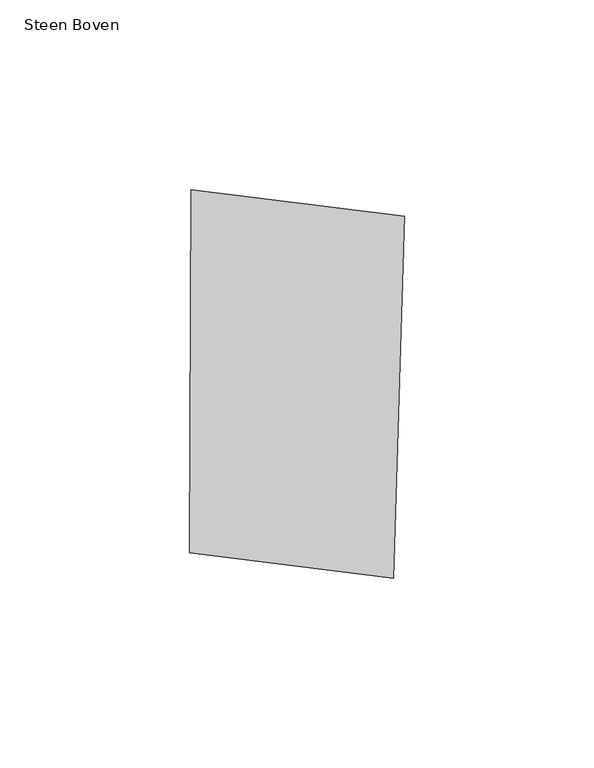
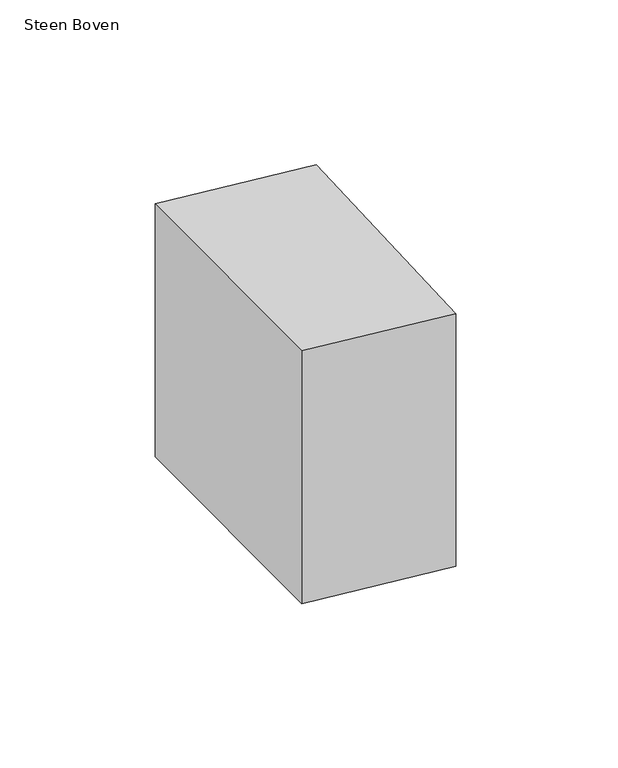
"""IFC4 building model written with IfcOpenShell, lengths in millimetres: proxy geometry, 00_GMA_steen_versie_4 : Steen Boven."""

import ifcopenshell
import ifcopenshell.guid

model = None  # the IFC model being written
_history = None  # IfcOwnerHistory: only IFC2X3 demands one
_inside = {}  # id of a spatial element -> (the spatial element, [elements in it])
_under = {}  # id of a project, library or spatial element -> (it, [spatial elements below it])
_declared = {}  # id of a project -> (the project, [libraries it declares])
_typed = {}  # id of a type object -> (the type object, [elements of that type])
_made_of = {}  # id of a material, layer set ... -> (it, [elements and type objects made of it])


def new_model(schema):
    """Start an empty IFC model of exactly this schema.

    Asked for "IFC4X3", IfcOpenShell would pick the latest addendum, in which some entities
    have other attributes; the version numbers below select the first issue.
    IFC2X3 requires an IfcOwnerHistory on every rooted entity: one is made here for all.
    """
    global model, _history
    if schema == "IFC4X3":
        model = ifcopenshell.file(schema_version=(4, 3, 0, 0))
    else:
        model = ifcopenshell.file(schema=schema)
    _inside.clear()
    _under.clear()
    _declared.clear()
    _typed.clear()
    _made_of.clear()
    _history = None
    if model.schema == "IFC2X3":
        org = make("IfcOrganization", Name="unknown")
        user = make(
            "IfcPersonAndOrganization",
            ThePerson=make("IfcPerson", FamilyName="unknown"),
            TheOrganization=org,
        )
        app = make(
            "IfcApplication",
            ApplicationDeveloper=org,
            Version="unknown",
            ApplicationFullName="unknown",
            ApplicationIdentifier="unknown",
        )
        _history = make(
            "IfcOwnerHistory",
            OwningUser=user,
            OwningApplication=app,
            ChangeAction="ADDED",
            CreationDate=0,
        )
    return model


def make(cls, **values):
    """One entity of the class cls with the attributes given. An attribute that is None is left unset."""
    return model.create_entity(
        cls, **{name: value for name, value in values.items() if value is not None}
    )


def rooted(cls, **values):
    """An entity with a GlobalId (a new one), such as an element, a storey or a relation."""
    return make(cls, GlobalId=ifcopenshell.guid.new(), OwnerHistory=_history, **values)


def si_unit(unit_type, name, prefix=None):
    """IfcSIUnit, for example si_unit("LENGTHUNIT", "METRE", prefix="MILLI")."""
    return make("IfcSIUnit", UnitType=unit_type, Prefix=prefix, Name=name)


def assignment(units):
    """IfcUnitAssignment: the units of a project."""
    return None if units is None else make("IfcUnitAssignment", Units=units)


def point(xyz):
    """IfcCartesianPoint."""
    return None if xyz is None else make("IfcCartesianPoint", Coordinates=xyz)


def direction(xyz):
    """IfcDirection."""
    return None if xyz is None else make("IfcDirection", DirectionRatios=xyz)


def frame(location, z_axis=None, x_axis=None):
    """IfcAxis2Placement3D, a coordinate frame: its origin and axes. An axis left out is left unset."""
    return make(
        "IfcAxis2Placement3D",
        Location=point(location),
        Axis=direction(z_axis),
        RefDirection=direction(x_axis),
    )


def origin():
    """The frame at (0, 0, 0) with its axes left unset."""
    return frame((0.0, 0.0, 0.0))


def origin_with_axes():
    """The frame at (0, 0, 0) with the z axis (0, 0, 1) and the x axis (1, 0, 0) written out."""
    return frame((0.0, 0.0, 0.0), z_axis=(0.0, 0.0, 1.0), x_axis=(1.0, 0.0, 0.0))


def place(relative_to, where):
    """IfcLocalPlacement: puts the frame where relative to a parent placement (None: the world)."""
    return make(
        "IfcLocalPlacement", PlacementRelTo=relative_to, RelativePlacement=where
    )


def context(
    kind, dimensions, precision=None, world=None, true_north=None, identifier=None
):
    """IfcGeometricRepresentationContext, for example the 3D "Model" context."""
    return make(
        "IfcGeometricRepresentationContext",
        ContextIdentifier=identifier,
        ContextType=kind,
        CoordinateSpaceDimension=dimensions,
        Precision=precision,
        WorldCoordinateSystem=world,
        TrueNorth=true_north,
    )


def project(units=None, contexts=None):
    """IfcProject with its units and contexts."""
    return rooted(
        "IfcProject",
        Name="project",
        RepresentationContexts=contexts,
        UnitsInContext=assignment(units),
    )


def spatial(cls, under=None, at=None, **own):
    """A site, building, storey or space (cls), placed at a placement, below another one or the project."""
    s = rooted(cls, ObjectPlacement=at, **own)
    if under is not None:
        _under.setdefault(under.id(), (under, []))[1].append(s)
    return s


def polyline(points):
    """IfcPolyline through the points."""
    return make("IfcPolyline", Points=[point(p) for p in points])


def outline(outer, holes=None, kind="AREA"):
    """IfcArbitraryClosedProfileDef: a profile drawn as a closed curve; with holes, ...WithVoids."""
    if holes is None:
        return make("IfcArbitraryClosedProfileDef", ProfileType=kind, OuterCurve=outer)
    return make(
        "IfcArbitraryProfileDefWithVoids",
        ProfileType=kind,
        OuterCurve=outer,
        InnerCurves=holes,
    )


def extrude(swept, where, along, depth):
    """IfcExtrudedAreaSolid: the profile swept, set in the frame where, extruded along a direction by depth."""
    return make(
        "IfcExtrudedAreaSolid",
        SweptArea=swept,
        Position=where,
        ExtrudedDirection=direction(along),
        Depth=depth,
    )


def shape(context_of_items, identifier, shape_type, items):
    """IfcShapeRepresentation: the items that make up one representation, for example the "Body"."""
    return make(
        "IfcShapeRepresentation",
        ContextOfItems=context_of_items,
        RepresentationIdentifier=identifier,
        RepresentationType=shape_type,
        Items=items,
    )


def source(mapping_origin, context_of_items, identifier, shape_type, items):
    """IfcRepresentationMap: a shape defined once, which mapped items show again and again."""
    return make(
        "IfcRepresentationMap",
        MappingOrigin=mapping_origin,
        MappedRepresentation=shape(context_of_items, identifier, shape_type, items),
    )


def transform(
    local_origin,
    x_axis=None,
    y_axis=None,
    z_axis=None,
    scale=None,
    scale2=None,
    scale3=None,
    uniform=True,
):
    """IfcCartesianTransformationOperator3D, or its non-uniform kind. x_axis, y_axis, z_axis: its Axis1, 2, 3."""
    if uniform:
        return make(
            "IfcCartesianTransformationOperator3D",
            Axis1=direction(x_axis),
            Axis2=direction(y_axis),
            LocalOrigin=point(local_origin),
            Scale=scale,
            Axis3=direction(z_axis),
        )
    return make(
        "IfcCartesianTransformationOperator3DnonUniform",
        Axis1=direction(x_axis),
        Axis2=direction(y_axis),
        LocalOrigin=point(local_origin),
        Scale=scale,
        Axis3=direction(z_axis),
        Scale2=scale2,
        Scale3=scale3,
    )


def mapped(mapping_source, mapping_target):
    """IfcMappedItem: shows the shape of a source again, moved by a transform."""
    return make(
        "IfcMappedItem", MappingSource=mapping_source, MappingTarget=mapping_target
    )


def made_of(thing, what):
    """Note that an element or type object is made of a material, layer set ...; save() writes the relation."""
    if what is not None:
        _made_of.setdefault(what.id(), (what, []))[1].append(thing)
    return thing


def element(
    cls,
    number,
    at=None,
    inside=None,
    cuts=None,
    type_object=None,
    material=None,
    context=None,
    identifier="Body",
    shape_type=None,
    held_by="IfcProductDefinitionShape",
    body=None,
    shapes=None,
    **own,
):
    """One element of the class cls, such as IfcWall. Its Tag is "e" and its number.

    at: its placement. inside: the storey or other place that contains it. cuts: it is an
    opening in that element (IfcRelVoidsElement). A single representation is given by context,
    identifier, shape_type and body (its items); several are given by shapes. held_by: the class
    of the entity that holds the representations. save() writes the other relations.
    """
    e = rooted(cls, Tag="e%d" % number, ObjectPlacement=at, **own)
    if body is not None:
        shapes = [shape(context, identifier, shape_type, body)]
    if shapes is not None:
        e.Representation = make(held_by, Representations=shapes)
    if inside is not None:
        _inside.setdefault(inside.id(), (inside, []))[1].append(e)
    if cuts is not None:
        rooted(
            "IfcRelVoidsElement", RelatingBuildingElement=cuts, RelatedOpeningElement=e
        )
    if type_object is not None:
        _typed.setdefault(type_object.id(), (type_object, []))[1].append(e)
    return made_of(e, material)


def aggregate(whole, parts):
    """IfcRelAggregates: a whole, such as a stair, and the parts it consists of."""
    return rooted("IfcRelAggregates", RelatingObject=whole, RelatedObjects=parts)


def save(model, path):
    """Write the relations noted so far, then the file.

    IfcRelAggregates (storeys below a building ...), IfcRelContainedInSpatialStructure (elements
    in a storey), IfcRelDefinesByType, IfcRelAssociatesMaterial and IfcRelDeclares: one each for
    every whole, place, type object, material and project.
    """
    for whole, parts in _under.values():
        aggregate(whole, parts)
    for where, things in _inside.values():
        rooted(
            "IfcRelContainedInSpatialStructure",
            RelatedElements=things,
            RelatingStructure=where,
        )
    for kind, things in _typed.values():
        rooted("IfcRelDefinesByType", RelatedObjects=things, RelatingType=kind)
    for what, things in _made_of.values():
        rooted("IfcRelAssociatesMaterial", RelatedObjects=things, RelatingMaterial=what)
    for by, libraries in _declared.values():
        rooted("IfcRelDeclares", RelatingContext=by, RelatedDefinitions=libraries)
    model.write(path)


def steen_boven_6cf3bcd0(model_context):
    return source(origin(), model_context, "Body", "SweptSolid", [
        extrude(outline(polyline([(102.1423558, 119.4078233), (99.1949074, 24.0176525), (45.4776731, 30.6984154), (45.9104462, 126.4137813), (102.1423558, 119.4078233)])), origin_with_axes(), (0.0, 0.0, 1.0), 100.0),
    ])


if __name__ == "__main__":
    model = new_model("IFC4")
    model_context = context("Model", 3, world=origin())
    ifc_project = project(units=[si_unit("LENGTHUNIT", "METRE", prefix="MILLI")], contexts=[model_context])
    site = spatial("IfcSite", under=ifc_project)
    building = spatial("IfcBuilding", under=site)
    placement = place(None, origin())
    steen_boven_shape = steen_boven_6cf3bcd0(model_context)
    element("IfcBuildingElementProxy", 1, Name="00_GMA_steen_versie_4 : Steen Boven", ObjectType="00_GMA_steen_versie_4 : Steen Boven", at=placement, inside=building, context=model_context, shape_type="MappedRepresentation", body=[
        mapped(steen_boven_shape, transform((0.0, 0.0, 0.0), x_axis=(1.0, 0.0, 0.0), y_axis=(0.0, 1.0, 0.0), z_axis=(0.0, 0.0, 1.0))),
    ])
    save(model, "model.ifc")

# Revit data of these elements
# Type "00_GMA_steen_versie_4 : Steen Boven"
#   StootVoegHalfBoven [instance default] = 5 mm
#   StootVoegHalf [instance default] = 5 mm
#   StootVoegBreedteOnder = 10 mm
#   StootVoegBreedteBoven = 10 mm
#   Steendikte = 100 mm
#   LintVoegOnderHalf = 5 mm
#   LintVoegOnder = 10 mm
#   LintVoegBovenHalf = 0 mm
#   LintVoegBoven = 0 mm
#   materiaal = none
#   MateriaalVoeg = none
#   Default Elevation = 0
